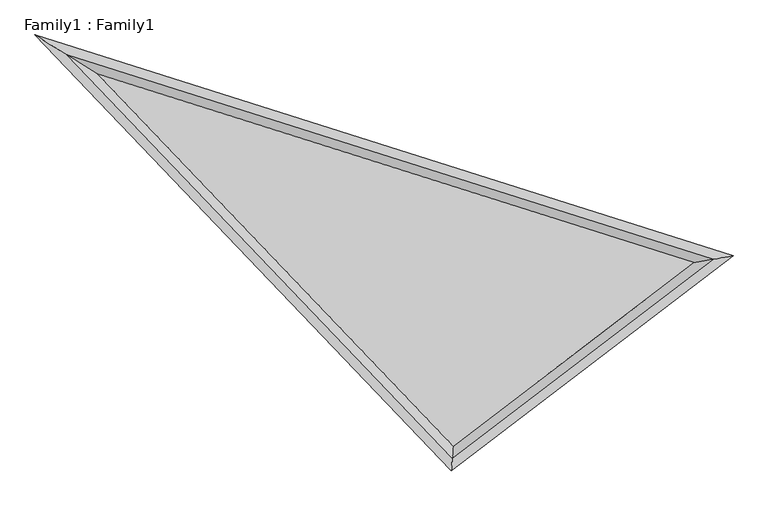
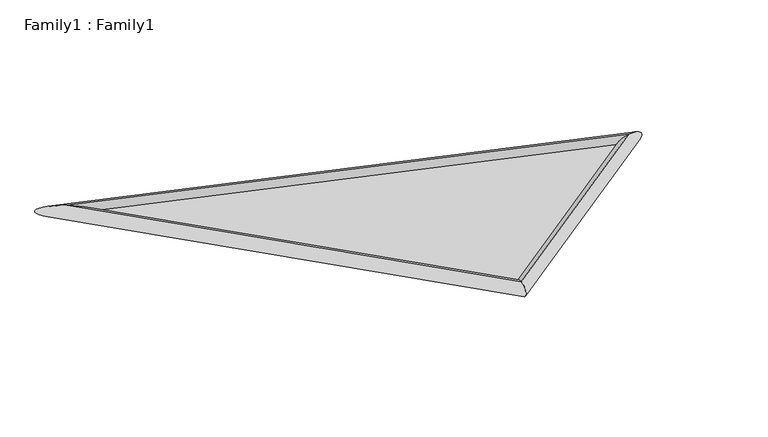
"""IFC4 building model written with IfcOpenShell, lengths in millimetres: proxy geometry, Family1 : Family1."""

from ifc_helpers import new_model, si_unit, frame, origin, origin_with_axes, place, context, project, spatial, polyline, ellipse_curve, outline, extrude, source, transform, mapped, element, save
from ifc_brep_helpers import cylinder_surface, advanced_brep


def family1_family1_e6d1cf26(model_context):
    return source(origin(), model_context, "Body", "SolidModel", [
        extrude(outline(polyline([(1365.4963109, -1677.8193886), (-2741.628814, 2619.7052994), (4143.0549541, 442.0552941), (1365.4963109, -1677.8193886)])), origin_with_axes(), (0.0, 0.0, 1.0), 34.1328789),
        advanced_brep(
        [(1365.4963109, -1677.8193886, 100.0), (1365.4963109, -1677.8193886, -100.0), (-2741.628814, 2619.7052994, -100.0), (-2741.628814, 2619.7052994, 100.0), (4143.0549541, 442.0552941, -100.0), (4143.0549541, 442.0552941, 100.0)],
        [
            (0, 1, ellipse_curve(frame((1365.4963109, -1677.8193886, 0.0), z_axis=(-0.9969539640662822, 0.07799226585069965, 0.0), x_axis=(-0.07799226585069975, -0.996953964066282, 0.0)), 134.1939882, 100.0)),
            (1, 2),
            (2, 3, ellipse_curve(frame((-2741.628814, 2619.7052994, 0.0), z_axis=(-0.5288095288307911, -0.8487405270268155, 0.0), x_axis=(0.8487405270268156, -0.5288095288307912, 0.0)), 402.8546968, 100.0)),
            (3, 0),
            (1, 0, ellipse_curve(frame((1365.4963109, -1677.8193886, 0.0), z_axis=(-0.9969539640662822, 0.07799226585069965, 0.0), x_axis=(-0.07799226585069975, -0.996953964066282, 0.0)), 134.1939882, 100.0)),
            (3, 2, ellipse_curve(frame((-2741.628814, 2619.7052994, 0.0), z_axis=(-0.5288095288307911, -0.8487405270268155, 0.0), x_axis=(0.8487405270268156, -0.5288095288307912, 0.0)), 402.8546968, 100.0)),
            (2, 4),
            (4, 5, ellipse_curve(frame((4143.0549541, 442.0552941, 0.0), z_axis=(-0.17192111831757625, 0.9851107191967986, 0.0), x_axis=(-0.9851107191967988, -0.1719211183175762, 0.0)), 216.918065, 100.0)),
            (5, 3),
            (5, 4, ellipse_curve(frame((4143.0549541, 442.0552941, 0.0), z_axis=(-0.17192111831757625, 0.9851107191967986, 0.0), x_axis=(-0.9851107191967988, -0.1719211183175762, 0.0)), 216.918065, 100.0)),
            (4, 1),
            (0, 5),
        ],
        [
            cylinder_surface(frame((1365.4963109, -1677.8193886, 0.0), z_axis=(0.6909106640905173, -0.7229401456870413, 0.0), x_axis=(-0.7229401456870413, -0.6909106640905173, 0.0)), 100.0),
            cylinder_surface(frame((-2741.628814, 2619.7052994, 0.0), z_axis=(-0.9534418114148439, 0.3015770419743209, 0.0), x_axis=(0.3015770419743209, 0.9534418114148439, 0.0)), 100.0),
            cylinder_surface(frame((4143.0549541, 442.0552941, 0.0), z_axis=(0.7949293165290278, 0.6067020535012988, 0.0), x_axis=(0.6067020535012988, -0.7949293165290278, 0.0)), 100.0),
        ],
        [
            (0, [[1, 2, 3, 4]]),
            (0, [[5, -4, 6, -2]]),
            (1, [[-3, 7, 8, 9]]),
            (1, [[-6, -9, 10, -7]]),
            (2, [[-8, 11, -1, 12]]),
            (2, [[-10, -12, -5, -11]]),
        ],
    ),
    ])


if __name__ == "__main__":
    model = new_model("IFC4")
    model_context = context("Model", 3, world=origin())
    ifc_project = project(units=[si_unit("LENGTHUNIT", "METRE", prefix="MILLI")], contexts=[model_context])
    site = spatial("IfcSite", under=ifc_project)
    building = spatial("IfcBuilding", under=site)
    placement = place(None, origin())
    family1_family1_shape = family1_family1_e6d1cf26(model_context)
    element("IfcBuildingElementProxy", 1, Name="Family1 : Family1", ObjectType="Family1 : Family1", at=placement, inside=building, context=model_context, shape_type="MappedRepresentation", body=[
        mapped(family1_family1_shape, transform((0.0, 0.0, 0.0), x_axis=(1.0, 0.0, 0.0), y_axis=(0.0, 1.0, 0.0), z_axis=(0.0, 0.0, 1.0))),
    ])
    save(model, "model.ifc")

# Revit data of these elements
# Type "Family1 : Family1"
#   Default Elevation = 0
# Element 1 (IfcBuildingElementProxy, "Family1 : Family1")
#   Materials on its faces: "Glass"
# Materials
#   "Glass": class "Glass", colour RGB 0 128 192, transparency 0.9, Description = "Soda Lime Glass", Cost = 0
